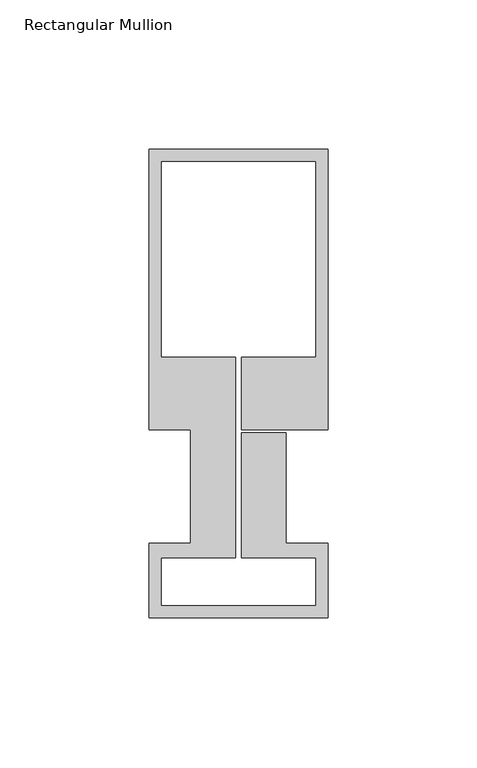
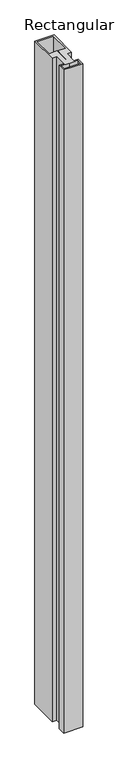
"""IFC4 building model written with IfcOpenShell, lengths in millimetres: member geometry, Rectangular Mullion : Schueco_FWS-60-SI_Mull_CovCap-20mm_Mull-85mm."""

from ifc_helpers import new_model, si_unit, frame, origin, place, context, project, spatial, polyline, outline, extrude, source, transform, mapped, element, save


def rectangular_mullion_dc96b6fd(model_context):
    return source(origin(), model_context, "Body", "SweptSolid", [
        extrude(outline(polyline([(-60.0, 132.0), (0.0, 132.0), (0.0, 38.0), (-29.0, 38.0), (-29.0, 62.3), (-4.0, 62.3), (-4.0, 128.0), (-56.0, 128.0), (-56.0, 62.3), (-31.0, 62.3), (-31.0, -5.0), (-56.0, -5.0), (-56.0, -21.0), (-4.0, -21.0), (-4.0, -5.0), (-29.0, -5.0), (-29.0, 37.0), (-14.0, 37.0), (-14.0, -0.1), (0.0, -0.1), (0.0, -25.0), (-60.0, -25.0), (-60.0, -0.1), (-46.0, -0.1), (-46.0, 38.0), (-60.0, 38.0), (-60.0, 132.0)])), frame((0.0, 0.0, -2200.0), z_axis=(0.0, 0.0, 1.0), x_axis=(1.0, 0.0, 0.0)), (0.0, 0.0, 1.0), 2200.0),
    ])


if __name__ == "__main__":
    model = new_model("IFC4")
    model_context = context("Model", 3, world=origin())
    ifc_project = project(units=[si_unit("LENGTHUNIT", "METRE", prefix="MILLI")], contexts=[model_context])
    site = spatial("IfcSite", under=ifc_project)
    building = spatial("IfcBuilding", under=site)
    placement = place(None, origin())
    rectangular_mullion_shape = rectangular_mullion_dc96b6fd(model_context)
    element("IfcMember", 1, ObjectType="Rectangular Mullion : Schueco_FWS-60-SI_Mull_CovCap-20mm_Mull-85mm", at=placement, inside=building, context=model_context, shape_type="MappedRepresentation", body=[
        mapped(rectangular_mullion_shape, transform((0.0, 0.0, 0.0), x_axis=(1.0, 0.0, 0.0), y_axis=(0.0, 1.0, 0.0), z_axis=(0.0, 0.0, 1.0))),
    ])
    save(model, "model.ifc")

# Revit data of these elements
# Type "Rectangular Mullion : Schueco_FWS-60-SI_Mull_CovCap-20mm_Mull-85mm"
#   Model = "FWS 60.SI"
#   Manufacturer = "Schueco International KG"
#   Type Comments = "Mullion"
#   Schueco thermal insulation standard = "Suitable for passive houses"
#   Burglar resistance = "RC 3"
#   Thermal insulation = "to 0.70 W/(m²K)"
#   built-in parameter 1007322 = 0.515092 (stored number, unit not read)
#   built-in parameter 1007321 = 0.0524934 (stored number, unit not read)
#   built-in parameter 1007320 = 0.0524934 (stored number, unit not read)
# Element 1 (IfcMember, "Rectangular Mullion : Schueco_FWS-60-SI_Mull_CovCap-20mm_Mull-85mm")
#   Materials on its faces: "Alu"
# Materials
#   "Alu": class "Glas", colour RGB 140 140 140, transparency 0
